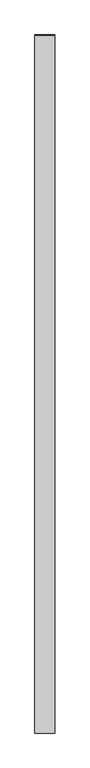
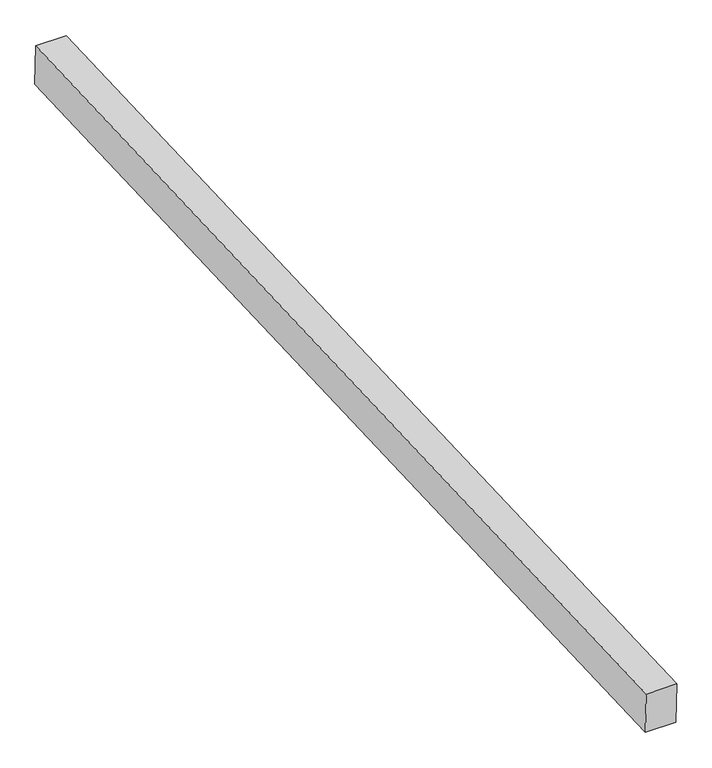
"""IFC4 building model written with IfcOpenShell, lengths in millimetres: proxy geometry, Generic Models 7:Generic Models 1:8:Generic Models 1:8 : Generic Models 7:Generic Models 1:337419:8 : Generic Models 7:Generic Models 1:8:Generic Models 1:8 : Generic Models 7:Generic Models 1:337419:315935."""

from ifc_helpers import new_model, si_unit, frame, origin, place, context, project, spatial, polyline, outline, extrude, source, transform, mapped, element, save


def generic_models_a0f8866c(model_context):
    return source(origin(), model_context, "Body", "SweptSolid", [
        extrude(outline(polyline([(-580626.555738, 3844.0209448), (-575753.6328438, 4047.0593987), (-575746.0659221, 3856.7093942), (-580618.6251193, 3653.6860944), (-580626.555738, 3844.0209448)])), frame((592439.511724, 0.0, 0.0), z_axis=(1.0, 0.0, 0.0), x_axis=(0.0, 1.0, 0.0)), (0.0, 0.0, 1.0), 139.7),
    ])


if __name__ == "__main__":
    model = new_model("IFC4")
    model_context = context("Model", 3, world=origin())
    ifc_project = project(units=[si_unit("LENGTHUNIT", "METRE", prefix="MILLI")], contexts=[model_context])
    site = spatial("IfcSite", under=ifc_project)
    building = spatial("IfcBuilding", under=site)
    placement = place(None, origin())
    generic_models_shape = generic_models_a0f8866c(model_context)
    element("IfcBuildingElementProxy", 1, Name="Generic Models 7:Generic Models 1:8:Generic Models 1:8 : Generic Models 7:Generic Models 1:337419:8 : Generic Models 7:Generic Models 1:8:Generic Models 1:8 : Generic Models 7:Generic Models 1:337419:315935", ObjectType="Generic Models 7:Generic Models 1:8:Generic Models 1:8 : Generic Models 7:Generic Models 1:337419:8 : Generic Models 7:Generic Models 1:8:Generic Models 1:8 : Generic Models 7:Generic Models 1:337419:315935", at=placement, inside=building, context=model_context, shape_type="MappedRepresentation", body=[
        mapped(generic_models_shape, transform((0.0, 0.0, 0.0), x_axis=(1.0, 0.0, 0.0), y_axis=(0.0, 1.0, 0.0), z_axis=(0.0, 0.0, 1.0))),
    ])
    save(model, "model.ifc")

# Revit data of these elements
# Type "Generic Models 7:Generic Models 1:8:Generic Models 1:8 : Generic Models 7:Generic Models 1:337419:8 : Generic Models 7:Generic Models 1:8:Generic Models 1:8 : Generic Models 7:Generic Models 1:337419:315935"
#   NameOverride = "Generic Models 7:Generic Models 1:8:Generic Models 1:8 : Generic Models 7:Generic Models 1:337419:315935"
#   ObjectTypeOverride = "Generic Models 1:8 : Generic Models 7:Generic Models 1:337419"
#   Reference = "Generic Models 1"
#   Tag = "315935"
# Element 1 (IfcBuildingElementProxy, "Generic Models 7:Generic Models 1:8:Generic Models 1:8 : Generic Models 7:Generic Models 1:337419:8 : Generic Models 7:Generic Models 1:8:Generic Models 1:8 : Generic Models 7:Generic Models 1:337419:315935")
#   Materials on its faces: "5 1/8\" X 7 1/2\" EXTERIOR GRADE GLULAM BEAMS (4'- 0 1/4\" O.C.)"
# Materials
#   "5 1/8\" X 7 1/2\" EXTERIOR GRADE GLULAM BEAMS (4'- 0 1/4\" O.C.)": class "Wood", colour RGB 183 134 68, transparency 0, Keynote = "M06181300.01", Description = "Pinus Echinata", Cost = 0
